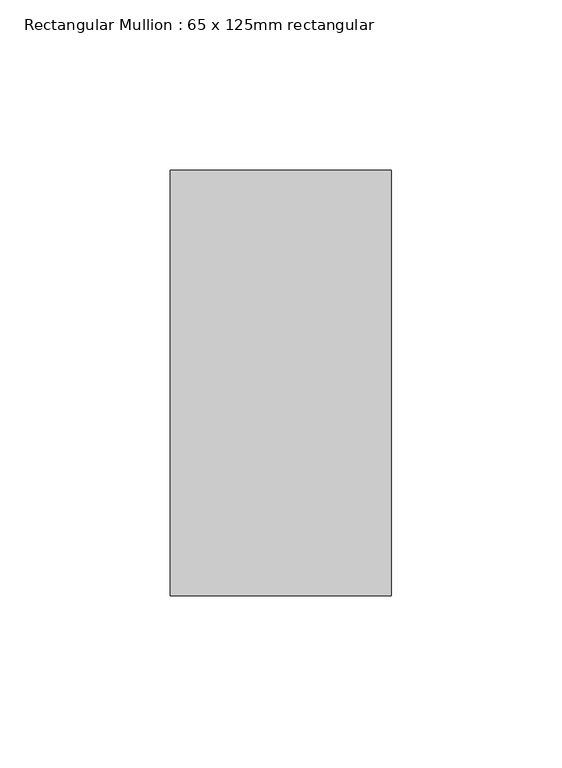
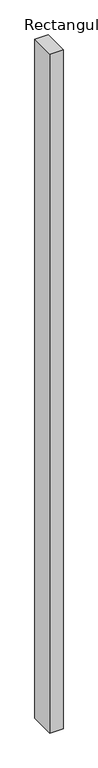
"""IFC4 building model written with IfcOpenShell, lengths in millimetres: member geometry, Rectangular Mullion : 65 x 125mm rectangular."""

from ifc_helpers import new_model, si_unit, frame, origin, place, context, project, spatial, polyline, outline, extrude, source, transform, mapped, element, save


def rectangular_mullion_65_x_125mm_rectangular_c6a61499(model_context):
    return source(origin(), model_context, "Body", "SweptSolid", [
        extrude(outline(polyline([(32.5, 62.5), (32.5, -62.5), (-32.5, -62.5), (-32.5, 62.5), (32.5, 62.5)])), frame((0.0, 0.0, -3500.0), z_axis=(0.0, 0.0, 1.0), x_axis=(1.0, 0.0, 0.0)), (0.0, 0.0, 1.0), 3500.0),
    ])


if __name__ == "__main__":
    model = new_model("IFC4")
    model_context = context("Model", 3, world=origin())
    ifc_project = project(units=[si_unit("LENGTHUNIT", "METRE", prefix="MILLI")], contexts=[model_context])
    site = spatial("IfcSite", under=ifc_project)
    building = spatial("IfcBuilding", under=site)
    placement = place(None, origin())
    rectangular_mullion_65_x_125mm_rectangular_shape = rectangular_mullion_65_x_125mm_rectangular_c6a61499(model_context)
    element("IfcMember", 1, ObjectType="Rectangular Mullion : 65 x 125mm rectangular", at=placement, inside=building, context=model_context, shape_type="MappedRepresentation", body=[
        mapped(rectangular_mullion_65_x_125mm_rectangular_shape, transform((0.0, 0.0, 0.0), x_axis=(1.0, 0.0, 0.0), y_axis=(0.0, 1.0, 0.0), z_axis=(0.0, 0.0, 1.0))),
    ])
    save(model, "model.ifc")

# Revit data of these elements
# Type "Rectangular Mullion : 65 x 125mm rectangular"
#   built-in parameter 1007304 = 0.410105 (stored number, unit not read)
#   built-in parameter 1007301 = 0.106627 (stored number, unit not read)
#   built-in parameter 1007300 = 0.106627 (stored number, unit not read)
# Element 1 (IfcMember, "Rectangular Mullion : 65 x 125mm rectangular")
#   Materials on its faces: "Aluminum"
# Materials
#   "Aluminum": class "Metal", colour RGB 244 245 246, transparency 0, Description = "Aluminum 6061", Cost = 0
